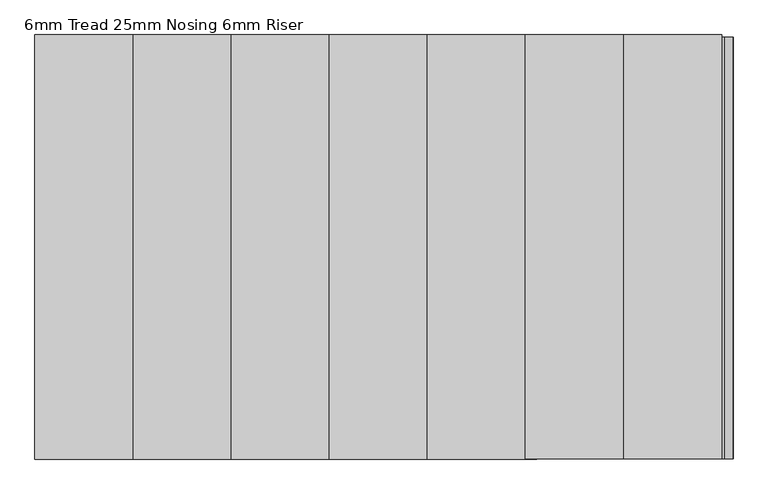
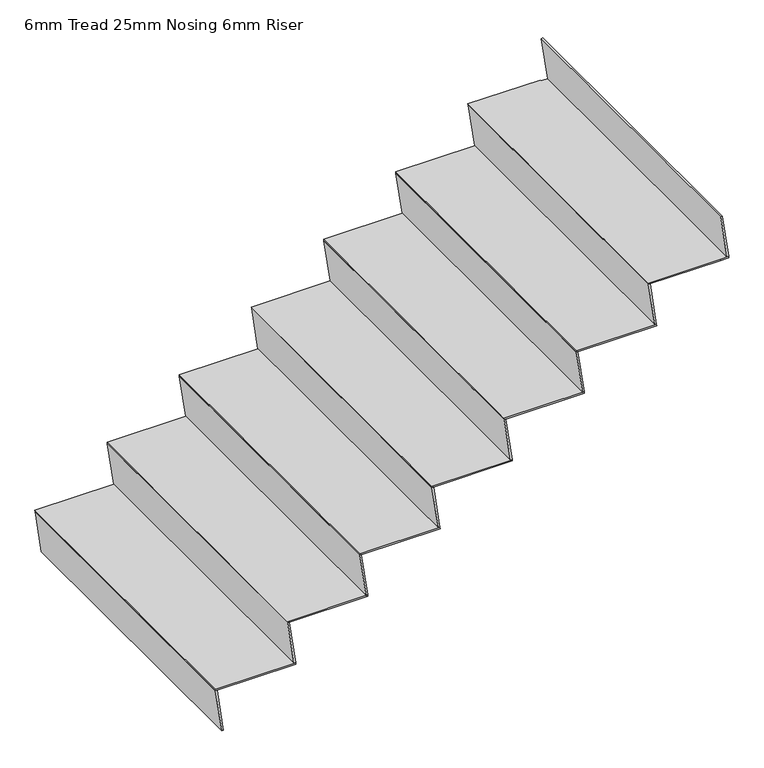
"""IFC4 building model written with IfcOpenShell, lengths in millimetres: stair flight geometry, 6mm Tread 25mm Nosing 6mm Riser."""

from ifc_helpers import new_model, si_unit, origin, place, context, project, spatial, faceted_brep, source, transform, mapped, element, save


def stair_flight_6mm_tread_25mm_nosing_6mm_riser_defb4d85(model_context):
    return source(origin(), model_context, "Body", "Brep", [
        faceted_brep([(-16043.9400908, 12030.4345331, 30764.7058824), (-16043.0900908, 12030.4345331, 30758.7058824), (-16043.0900908, 13220.4345331, 30758.7058824), (-16043.9400908, 13220.4345331, 30764.7058824), (-16350.0, 13220.4345331, 30764.7058824), (-16350.0, 12030.4345331, 30764.7058824), (-16349.15, 12030.4345331, 30758.7058824), (-16349.15, 13220.4345331, 30758.7058824)], [[[0, 1, 2, 3]], [[3, 4, 5, 0]], [[2, 1, 6, 7]], [[4, 3, 2, 7]], [[0, 5, 6, 1]], [[5, 4, 7, 6]]]),
        faceted_brep([(-16349.15, 12030.4345331, 30758.7058824), (-16325.0, 12030.4345331, 30588.2352941), (-16318.9400908, 12030.4345331, 30588.2352941), (-16343.0900908, 12030.4345331, 30758.7058824), (-16349.15, 13220.4345331, 30758.7058824), (-16343.0900908, 13220.4345331, 30758.7058824), (-16318.9400908, 13220.4345331, 30588.2352941), (-16325.0, 13220.4345331, 30588.2352941)], [[[0, 1, 2, 3]], [[4, 5, 6, 7]], [[1, 0, 4, 7]], [[2, 1, 7, 6]], [[3, 2, 6, 5]], [[0, 3, 5, 4]]]),
        faceted_brep([(-16074.15, 12030.4345331, 30935.1764706), (-16050.0, 12030.4345331, 30764.7058824), (-16043.9400908, 12030.4345331, 30764.7058824), (-16068.0900908, 12030.4345331, 30935.1764706), (-16074.15, 13220.4345331, 30935.1764706), (-16068.0900908, 13220.4345331, 30935.1764706), (-16043.9400908, 13220.4345331, 30764.7058824), (-16050.0, 13220.4345331, 30764.7058824)], [[[0, 1, 2, 3]], [[4, 5, 6, 7]], [[1, 0, 4, 7]], [[2, 1, 7, 6]], [[3, 2, 6, 5]], [[0, 3, 5, 4]]]),
        faceted_brep([(-15768.9400908, 13220.4345331, 30941.1764706), (-16075.0, 13220.4345331, 30941.1764706), (-16075.0, 12030.4345331, 30941.1764706), (-15768.9400908, 12030.4345331, 30941.1764706), (-15768.0900908, 13220.4345331, 30935.1764706), (-15768.0900908, 12030.4345331, 30935.1764706), (-16074.15, 12030.4345331, 30935.1764706), (-16074.15, 13220.4345331, 30935.1764706)], [[[0, 1, 2, 3]], [[4, 5, 6, 7]], [[1, 0, 4, 7]], [[3, 2, 6, 5]], [[3, 5, 4, 0]], [[2, 1, 7, 6]]]),
        faceted_brep([(-15799.15, 12030.4345331, 31111.6470588), (-15775.0, 12030.4345331, 30941.1764706), (-15768.9400908, 12030.4345331, 30941.1764706), (-15793.0900908, 12030.4345331, 31111.6470588), (-15799.15, 13220.4345331, 31111.6470588), (-15793.0900908, 13220.4345331, 31111.6470588), (-15768.9400908, 13220.4345331, 30941.1764706), (-15775.0, 13220.4345331, 30941.1764706)], [[[0, 1, 2, 3]], [[4, 5, 6, 7]], [[1, 0, 4, 7]], [[2, 1, 7, 6]], [[3, 2, 6, 5]], [[0, 3, 5, 4]]]),
        faceted_brep([(-15493.9400908, 13220.4345331, 31117.6470588), (-15800.0, 13220.4345331, 31117.6470588), (-15800.0, 12030.4345331, 31117.6470588), (-15493.9400908, 12030.4345331, 31117.6470588), (-15493.0900908, 13220.4345331, 31111.6470588), (-15493.0900908, 12030.4345331, 31111.6470588), (-15799.15, 12030.4345331, 31111.6470588), (-15799.15, 13220.4345331, 31111.6470588)], [[[0, 1, 2, 3]], [[4, 5, 6, 7]], [[1, 0, 4, 7]], [[3, 2, 6, 5]], [[3, 5, 4, 0]], [[2, 1, 7, 6]]]),
        faceted_brep([(-15524.15, 12030.4345331, 31288.1176471), (-15500.0, 12030.4345331, 31117.6470588), (-15493.9400908, 12030.4345331, 31117.6470588), (-15518.0900908, 12030.4345331, 31288.1176471), (-15524.15, 13220.4345331, 31288.1176471), (-15518.0900908, 13220.4345331, 31288.1176471), (-15493.9400908, 13220.4345331, 31117.6470588), (-15500.0, 13220.4345331, 31117.6470588)], [[[0, 1, 2, 3]], [[4, 5, 6, 7]], [[1, 0, 4, 7]], [[2, 1, 7, 6]], [[3, 2, 6, 5]], [[0, 3, 5, 4]]]),
        faceted_brep([(-15218.9400908, 13220.4345331, 31294.1176471), (-15525.0, 13220.4345331, 31294.1176471), (-15525.0, 12030.4345331, 31294.1176471), (-15218.9400908, 12030.4345331, 31294.1176471), (-15218.0900908, 13220.4345331, 31288.1176471), (-15218.0900908, 12030.4345331, 31288.1176471), (-15524.15, 12030.4345331, 31288.1176471), (-15524.15, 13220.4345331, 31288.1176471)], [[[0, 1, 2, 3]], [[4, 5, 6, 7]], [[1, 0, 4, 7]], [[3, 2, 6, 5]], [[3, 5, 4, 0]], [[2, 1, 7, 6]]]),
        faceted_brep([(-15249.15, 12030.4345331, 31464.5882353), (-15225.0, 12030.4345331, 31294.1176471), (-15218.9400908, 12030.4345331, 31294.1176471), (-15243.0900908, 12030.4345331, 31464.5882353), (-15249.15, 13220.4345331, 31464.5882353), (-15243.0900908, 13220.4345331, 31464.5882353), (-15218.9400908, 13220.4345331, 31294.1176471), (-15225.0, 13220.4345331, 31294.1176471)], [[[0, 1, 2, 3]], [[4, 5, 6, 7]], [[1, 0, 4, 7]], [[2, 1, 7, 6]], [[3, 2, 6, 5]], [[0, 3, 5, 4]]]),
        faceted_brep([(-14943.9400908, 13220.4345331, 31470.5882353), (-15250.0, 13220.4345331, 31470.5882353), (-15250.0, 12030.4345331, 31470.5882353), (-14943.9400908, 12030.4345331, 31470.5882353), (-14943.0900908, 13220.4345331, 31464.5882353), (-14943.0900908, 12030.4345331, 31464.5882353), (-15249.15, 12030.4345331, 31464.5882353), (-15249.15, 13220.4345331, 31464.5882353)], [[[0, 1, 2, 3]], [[4, 5, 6, 7]], [[1, 0, 4, 7]], [[3, 2, 6, 5]], [[3, 5, 4, 0]], [[2, 1, 7, 6]]]),
        faceted_brep([(-14974.15, 12030.4345331, 31641.0588235), (-14950.0, 12030.4345331, 31470.5882353), (-14943.9400908, 12030.4345331, 31470.5882353), (-14968.0900908, 12030.4345331, 31641.0588235), (-14974.15, 13220.4345331, 31641.0588235), (-14968.0900908, 13220.4345331, 31641.0588235), (-14943.9400908, 13220.4345331, 31470.5882353), (-14950.0, 13220.4345331, 31470.5882353)], [[[0, 1, 2, 3]], [[4, 5, 6, 7]], [[1, 0, 4, 7]], [[2, 1, 7, 6]], [[3, 2, 6, 5]], [[0, 3, 5, 4]]]),
        faceted_brep([(-14668.9400908, 13220.4345331, 31647.0588235), (-14975.0, 13220.4345331, 31647.0588235), (-14975.0, 12030.4345331, 31647.0588235), (-14668.9400908, 12030.4345331, 31647.0588235), (-14668.0900908, 13220.4345331, 31641.0588235), (-14668.0900908, 12030.4345331, 31641.0588235), (-14974.15, 12030.4345331, 31641.0588235), (-14974.15, 13220.4345331, 31641.0588235)], [[[0, 1, 2, 3]], [[4, 5, 6, 7]], [[1, 0, 4, 7]], [[3, 2, 6, 5]], [[3, 5, 4, 0]], [[2, 1, 7, 6]]]),
        faceted_brep([(-14424.15, 12030.4345331, 31994.0), (-14400.0, 12030.4345331, 31823.5294118), (-14393.9400908, 12030.4345331, 31823.5294118), (-14418.0900908, 12030.4345331, 31994.0), (-14424.15, 13214.4345331, 31994.0), (-14418.0900908, 13214.4345331, 31994.0), (-14393.9400908, 13214.4345331, 31823.5294118), (-14400.0, 13214.4345331, 31823.5294118)], [[[0, 1, 2, 3]], [[4, 5, 6, 7]], [[1, 0, 4, 7]], [[2, 1, 7, 6]], [[3, 2, 6, 5]], [[0, 3, 5, 4]]]),
        faceted_brep([(-14699.15, 12030.4345331, 31817.5294118), (-14675.0, 12030.4345331, 31647.0588235), (-14668.9400908, 12030.4345331, 31647.0588235), (-14693.0900908, 12030.4345331, 31817.5294118), (-14699.15, 13220.4345331, 31817.5294118), (-14693.0900908, 13220.4345331, 31817.5294118), (-14668.9400908, 13220.4345331, 31647.0588235), (-14675.0, 13220.4345331, 31647.0588235)], [[[0, 1, 2, 3]], [[4, 5, 6, 7]], [[1, 0, 4, 7]], [[2, 1, 7, 6]], [[3, 2, 6, 5]], [[0, 3, 5, 4]]]),
        faceted_brep([(-14393.9400908, 13214.4345331, 31823.5294118), (-14425.0, 13214.4345331, 31823.5294118), (-14425.0, 13220.4345331, 31823.5294118), (-14700.0, 13220.4345331, 31823.5294118), (-14700.0, 12030.4345331, 31823.5294118), (-14425.0, 12030.4345331, 31823.5294118), (-14393.9400908, 12030.4345331, 31823.5294118), (-14425.0, 13220.4345331, 31817.5294118), (-14425.0, 13214.4345331, 31817.5294118), (-14393.0900908, 13214.4345331, 31817.5294118), (-14393.0900908, 12030.4345331, 31817.5294118), (-14425.0, 12030.4345331, 31817.5294118), (-14699.15, 12030.4345331, 31817.5294118), (-14699.15, 13220.4345331, 31817.5294118)], [[[0, 1, 2, 3, 4, 5, 6]], [[7, 8, 9, 10, 11, 12, 13]], [[1, 0, 9, 8]], [[2, 1, 8, 7]], [[3, 2, 7, 13]], [[5, 4, 12, 11]], [[6, 5, 11, 10]], [[6, 10, 9, 0]], [[4, 3, 13, 12]]]),
    ])


if __name__ == "__main__":
    model = new_model("IFC4")
    model_context = context("Model", 3, world=origin())
    ifc_project = project(units=[si_unit("LENGTHUNIT", "METRE", prefix="MILLI")], contexts=[model_context])
    site = spatial("IfcSite", under=ifc_project)
    building = spatial("IfcBuilding", under=site)
    placement = place(None, origin())
    stair_flight_6mm_tread_25mm_nosing_6mm_riser_shape = stair_flight_6mm_tread_25mm_nosing_6mm_riser_defb4d85(model_context)
    element("IfcStairFlight", 1, ObjectType="6mm Tread 25mm Nosing 6mm Riser", at=placement, inside=building, context=model_context, shape_type="MappedRepresentation", body=[
        mapped(stair_flight_6mm_tread_25mm_nosing_6mm_riser_shape, transform((0.0, 0.0, 0.0), x_axis=(1.0, 0.0, 0.0), y_axis=(0.0, 1.0, 0.0), z_axis=(0.0, 0.0, 1.0))),
    ])
    save(model, "model.ifc")

# Revit data of these elements
# Element 1 (IfcStairFlight, "6mm Tread 25mm Nosing 6mm Riser")
#   Materials on its faces: "Steel, Paint Finish, Dark Gray"
# Materials
#   "Steel, Paint Finish, Dark Gray": class "Metal", colour RGB 89 89 89, transparency 0, Description = "Steel, paint finish, dark gray, glossy", Cost = 0
